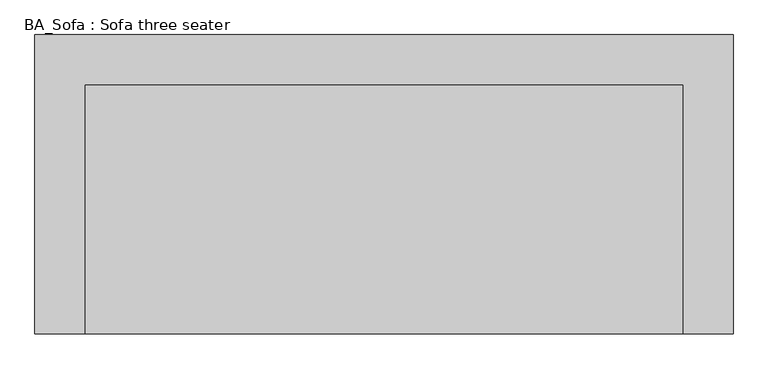
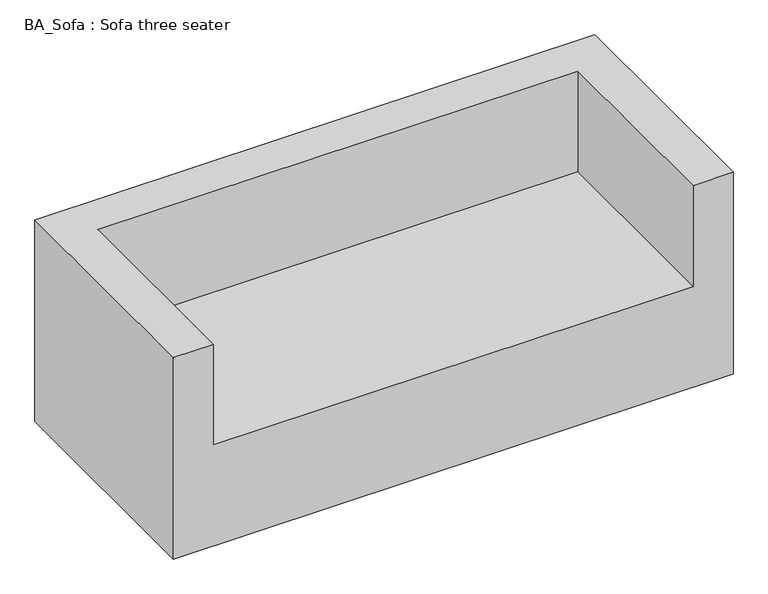
"""IFC4 building model written with IfcOpenShell, lengths in millimetres: furniture geometry, BA_Sofa : Sofa three seater."""

from ifc_helpers import new_model, si_unit, origin, place, context, project, spatial, faceted_brep, source, transform, mapped, element, save


def ba_sofa_sofa_three_seater_9d5b51f5(model_context):
    return source(origin(), model_context, "Body", "Brep", [
        faceted_brep([(1050.0, 450.0, 800.0), (-1050.0, 450.0, 800.0), (-1050.0, -450.0, 800.0), (-900.0, -450.0, 800.0), (-900.0, 300.0, 800.0), (900.0, 300.0, 800.0), (900.0, -450.0, 800.0), (1050.0, -450.0, 800.0), (1050.0, 450.0, 0.0), (1050.0, -450.0, 0.0), (-1050.0, -450.0, 0.0), (-1050.0, 450.0, 0.0), (900.0, -450.0, 400.0), (-900.0, -450.0, 400.0), (-900.0, 300.0, 400.0), (900.0, 300.0, 400.0)], [[[0, 1, 2, 3, 4, 5, 6, 7]], [[8, 9, 10, 11]], [[1, 0, 8, 11]], [[2, 1, 11, 10]], [[3, 2, 10, 9, 7, 6, 12, 13]], [[4, 3, 13, 14]], [[5, 4, 14, 15]], [[6, 5, 15, 12]], [[0, 7, 9, 8]], [[13, 12, 15, 14]]]),
    ])


if __name__ == "__main__":
    model = new_model("IFC4")
    model_context = context("Model", 3, world=origin())
    ifc_project = project(units=[si_unit("LENGTHUNIT", "METRE", prefix="MILLI")], contexts=[model_context])
    site = spatial("IfcSite", under=ifc_project)
    building = spatial("IfcBuilding", under=site)
    placement = place(None, origin())
    ba_sofa_sofa_three_seater_shape = ba_sofa_sofa_three_seater_9d5b51f5(model_context)
    element("IfcFurniture", 1, ObjectType="BA_Sofa : Sofa three seater", at=placement, inside=building, context=model_context, shape_type="MappedRepresentation", body=[
        mapped(ba_sofa_sofa_three_seater_shape, transform((0.0, 0.0, 0.0), x_axis=(1.0, 0.0, 0.0), y_axis=(0.0, 1.0, 0.0), z_axis=(0.0, 0.0, 1.0))),
    ])
    save(model, "model.ifc")

# Revit data of these elements
# Type "BA_Sofa : Sofa three seater"
#   height = 800 mm
#   width = 900 mm
#   length = 2100 mm
#   Default Elevation = 0
# Element 1 (IfcFurniture, "BA_Sofa : Sofa three seater")
#   Materials on its faces: "Default"
# Materials
#   "Default": class "Generic", colour RGB 255 255 255, transparency 0, Cost = 0
